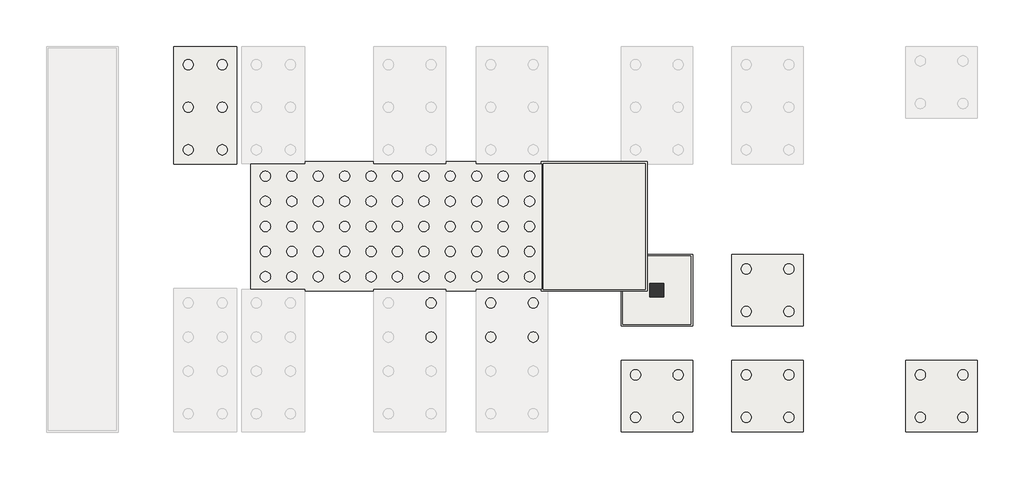
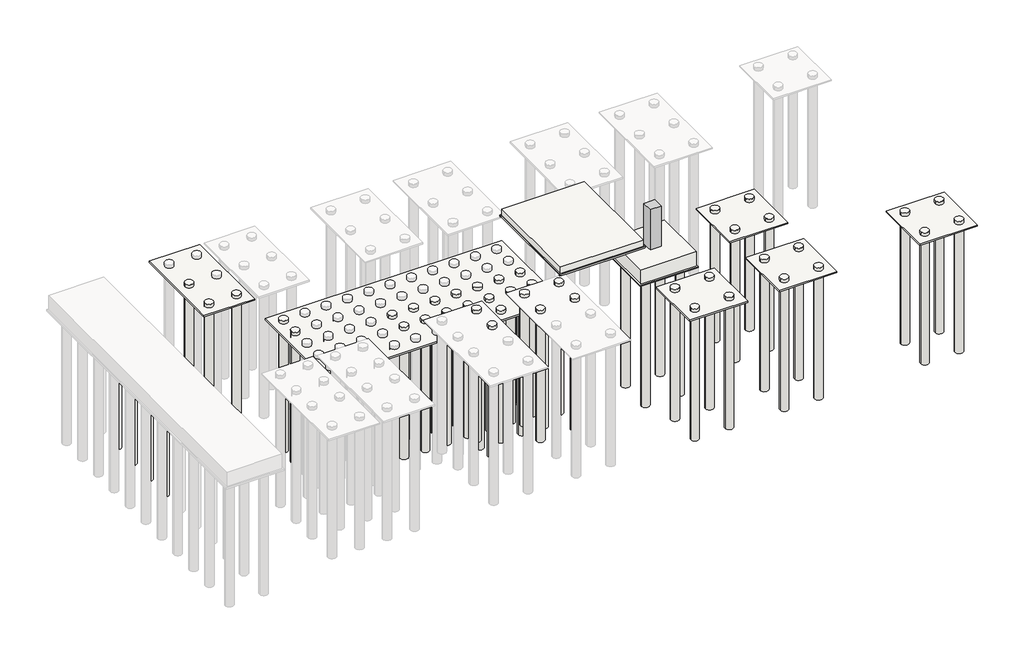
# One storey, part 2 of 3: 63 slabs, 1 column.
"""IFC4 building model written with IfcOpenShell, lengths in millimetres."""

from ifc_helpers import new_model, si_unit, point, frame, frame_2d, origin, place, context, project, spatial, polyline, circle_curve, trimmed, segment, composite_curve, outline, extrude, faceted_brep, element, save

model = new_model("IFC4")

# Units and contexts
model_context = context("Model", 3, world=origin())
ifc_project = project(units=[si_unit("LENGTHUNIT", "METRE", prefix="MILLI")], contexts=[model_context])

# Site, building, storey
site = spatial("IfcSite", under=ifc_project)
building = spatial("IfcBuilding", under=site)
storey = spatial("IfcBuildingStorey", under=building, Name="B.O.F(FDN)", Elevation=-2500.0279945)

# Column
placement = place(None, origin())
element("IfcColumn", 1, ObjectType="RC_Pedestal : H_SC_ACC_PED_W800xL800", at=placement, inside=storey, context=model_context, shape_type="SweptSolid", body=[
    extrude(outline(polyline([(33894.0, 26599.5208589), (33094.0, 26599.5208589), (33094.0, 27399.5208589), (33894.0, 27399.5208589), (33894.0, 26599.5208589)])), frame((0.0, 0.0, -2500.0279945), z_axis=(0.0, 0.0, 1.0), x_axis=(1.0, 0.0, 0.0)), (0.0, 0.0, 1.0), 3100.0),
])

# Slabs
element("IfcSlab", 2, ObjectType="H_SF_ACP_Pit Slab T500", at=placement, inside=storey, context=model_context, shape_type="Brep", body=[
    faceted_brep([(26830.0, 34449.5208589, -2400.0279945), (32830.0, 34449.5208589, -2400.0279945), (32830.0, 27049.5208589, -2400.0279945), (26830.0, 27049.5208589, -2400.0279945), (26830.0, 34449.5208589, -1900.0279945), (26830.0, 34059.5208589, -1900.0279945), (26830.0, 27439.5208589, -1900.0279945), (26830.0, 27049.5208589, -1900.0279945), (32830.0, 27049.5208589, -1900.0279945), (32830.0, 27439.5208589, -1900.0279945), (32830.0, 34059.5208589, -1900.0279945), (32830.0, 34449.5208589, -1900.0279945)], [[[0, 1, 2, 3]], [[4, 5, 6, 7, 8, 9, 10, 11]], [[1, 0, 4, 11]], [[2, 1, 11, 10, 9, 8]], [[3, 2, 8, 7]], [[0, 3, 7, 6, 5, 4]]]),
])
element("IfcSlab", 3, ObjectType="H_SF_ACF_Lean_T100", at=placement, inside=storey, context=model_context, shape_type="SweptSolid", body=[
    extrude(outline(polyline([(48115.0, 22879.5208589), (52315.0, 22879.5208589), (52315.0, 18679.5208589), (48115.0, 18679.5208589), (48115.0, 22879.5208589)])), frame((0.0, 0.0, -2600.0279945), z_axis=(0.0, 0.0, 1.0), x_axis=(1.0, 0.0, 0.0)), (0.0, 0.0, 1.0), 100.0),
])
element("IfcSlab", 4, ObjectType="H_SF_ACF_Lean_T100", at=placement, inside=storey, context=model_context, shape_type="SweptSolid", body=[
    extrude(outline(polyline([(5150.0, 41319.5208589), (8850.0, 41319.5208589), (8850.0, 34399.5208589), (5150.0, 34399.5208589), (5150.0, 41319.5208589)])), frame((0.0, 0.0, -2600.0279945), z_axis=(0.0, 0.0, 1.0), x_axis=(1.0, 0.0, 0.0)), (0.0, 0.0, 1.0), 100.0),
])
element("IfcSlab", 5, ObjectType="H_SF_ACF_Lean_T100", at=placement, inside=storey, context=model_context, shape_type="SweptSolid", body=[
    extrude(outline(polyline([(31400.0, 24899.5208589), (31400.0, 29099.5208589), (35600.0, 29099.5208589), (35600.0, 24899.5208589), (31400.0, 24899.5208589)])), frame((0.0, 0.0, -3700.0279945), z_axis=(0.0, 0.0, 1.0), x_axis=(1.0, 0.0, 0.0)), (0.0, 0.0, 1.0), 100.0),
])
element("IfcSlab", 6, ObjectType="H_SF_ACF_Lean_T100", at=placement, inside=storey, context=model_context, shape_type="Brep", body=[
    faceted_brep([(26730.0, 34549.5208589, -2500.0279945), (27000.0, 34549.5208589, -2500.0279945), (31500.0, 34549.5208589, -2500.0279945), (32930.0, 34549.5208589, -2500.0279945), (32930.0, 34499.5208589, -2500.0279945), (32930.0, 26949.5208589, -2500.0279945), (27000.0, 26949.5208589, -2500.0279945), (26730.0, 26949.5208589, -2500.0279945), (26730.0, 26999.5208589, -2500.0279945), (26730.0, 27049.5208589, -2500.0279945), (26780.0, 27049.5208589, -2500.0279945), (26780.0, 34449.5208589, -2500.0279945), (26730.0, 34449.5208589, -2500.0279945), (26730.0, 34499.5208589, -2500.0279945), (32930.0, 34549.5208589, -2400.0279945), (31500.0, 34549.5208589, -2400.0279945), (27000.0, 34549.5208589, -2400.0279945), (26730.0, 34549.5208589, -2400.0279945), (26730.0, 34499.5208589, -2400.0279945), (26730.0, 34449.5208589, -2400.0279945), (26780.0, 34449.5208589, -2400.0279945), (26780.0, 27049.5208589, -2400.0279945), (26730.0, 27049.5208589, -2400.0279945), (26730.0, 26999.5208589, -2400.0279945), (26730.0, 26949.5208589, -2400.0279945), (27000.0, 26949.5208589, -2400.0279945), (32930.0, 26949.5208589, -2400.0279945), (32930.0, 34499.5208589, -2400.0279945)], [[[0, 1, 2, 3, 4, 5, 6, 7, 8, 9, 10, 11, 12, 13]], [[14, 15, 16, 17, 18, 19, 20, 21, 22, 23, 24, 25, 26, 27]], [[3, 2, 1, 0, 17, 16, 15, 14]], [[5, 4, 3, 14, 27, 26]], [[7, 6, 5, 26, 25, 24]], [[17, 0, 13, 12, 19, 18]], [[7, 24, 23, 22, 9, 8]], [[20, 11, 10, 21]], [[21, 10, 9, 22]], [[11, 20, 19, 12]]]),
])
element("IfcSlab", 7, ObjectType="H_SF_ACF_Lean_T100", at=placement, inside=storey, context=model_context, shape_type="SweptSolid", body=[
    extrude(outline(polyline([(9680.0, 26949.5208589), (9680.0, 34549.5208589), (26880.0, 34549.5208589), (26880.0, 26949.5208589), (9680.0, 26949.5208589)])), frame((0.0, 0.0, -4500.0279945), z_axis=(0.0, 0.0, 1.0), x_axis=(1.0, 0.0, 0.0)), (0.0, 0.0, 1.0), 100.0),
])
element("IfcSlab", 8, ObjectType="H_SF_ACF_Lean_T100", at=placement, inside=storey, context=model_context, shape_type="SweptSolid", body=[
    extrude(outline(polyline([(37900.0, 22879.5208589), (42100.0, 22879.5208589), (42100.0, 18679.5208589), (37900.0, 18679.5208589), (37900.0, 22879.5208589)])), frame((0.0, 0.0, -2600.0279945), z_axis=(0.0, 0.0, 1.0), x_axis=(1.0, 0.0, 0.0)), (0.0, 0.0, 1.0), 100.0),
])
element("IfcSlab", 9, ObjectType="H_SF_ACF_Lean_T100", at=placement, inside=storey, context=model_context, shape_type="SweptSolid", body=[
    extrude(outline(polyline([(31400.0, 22879.5208589), (35600.0, 22879.5208589), (35600.0, 18679.5208589), (31400.0, 18679.5208589), (31400.0, 22879.5208589)])), frame((0.0, 0.0, -2600.0279945), z_axis=(0.0, 0.0, 1.0), x_axis=(1.0, 0.0, 0.0)), (0.0, 0.0, 1.0), 100.0),
])
element("IfcSlab", 10, ObjectType="H_SF_ACF_Lean_T100", at=placement, inside=storey, context=model_context, shape_type="SweptSolid", body=[
    extrude(outline(polyline([(37900.0, 29099.5208589), (42100.0, 29099.5208589), (42100.0, 24899.5208589), (37900.0, 24899.5208589), (37900.0, 29099.5208589)])), frame((0.0, 0.0, -2600.0279945), z_axis=(0.0, 0.0, 1.0), x_axis=(1.0, 0.0, 0.0)), (0.0, 0.0, 1.0), 100.0),
])
element("IfcSlab", 11, ObjectType="Foundation Rectangular(Non-Pile) : H_SF_ACF_W4000xL4000xT1100_Protection", at=placement, inside=storey, context=model_context, shape_type="SweptSolid", body=[
    extrude(outline(polyline([(35500.0, 28999.5208589), (35500.0, 24999.5208589), (31500.0, 24999.5208589), (31500.0, 28999.5208589), (35500.0, 28999.5208589)])), frame((0.0, 0.0, -3600.0279945), z_axis=(0.0, 0.0, 1.0), x_axis=(1.0, 0.0, 0.0)), (0.0, 0.0, 1.0), 1100.0),
])
element("IfcSlab", 12, ObjectType="Pile : H_SF_API_Steel Pile D508x12t_L10m", at=placement, inside=storey, context=model_context, shape_type="SweptSolid", body=[
    extrude(outline(composite_curve([segment(trimmed(circle_curve(frame_2d((1035.0, 38249.5208589)), 300.0), [point((1335.0, 38249.5208589))], [point((735.0, 38249.5208589))], False, "CARTESIAN"), True, "CONTINUOUS"), segment(trimmed(circle_curve(frame_2d((1035.0, 38249.5208589)), 300.0), [point((735.0, 38249.5208589))], [point((1335.0, 38249.5208589))], False, "CARTESIAN"), True, "CONTINUOUS")], self_intersect=False)), frame((0.0, 0.0, -13500.0279945), z_axis=(0.0, 0.0, 1.0), x_axis=(1.0, 0.0, 0.0)), (0.0, 0.0, 1.0), 10150.0),
])
element("IfcSlab", 13, ObjectType="Pile : H_SF_API_Steel Pile D508x12t_L10m", at=placement, inside=storey, context=model_context, shape_type="SweptSolid", body=[
    extrude(outline(composite_curve([segment(trimmed(circle_curve(frame_2d((1035.0, 36249.5208589)), 300.0), [point((1335.0, 36249.5208589))], [point((735.0, 36249.5208589))], False, "CARTESIAN"), True, "CONTINUOUS"), segment(trimmed(circle_curve(frame_2d((1035.0, 36249.5208589)), 300.0), [point((735.0, 36249.5208589))], [point((1335.0, 36249.5208589))], False, "CARTESIAN"), True, "CONTINUOUS")], self_intersect=False)), frame((0.0, 0.0, -13500.0279945), z_axis=(0.0, 0.0, 1.0), x_axis=(1.0, 0.0, 0.0)), (0.0, 0.0, 1.0), 10150.0),
])
element("IfcSlab", 14, ObjectType="Pile : H_SF_API_Steel Pile D508x12t_L10m", at=placement, inside=storey, context=model_context, shape_type="SweptSolid", body=[
    extrude(outline(composite_curve([segment(trimmed(circle_curve(frame_2d((1035.0, 34249.5208589)), 300.0), [point((1335.0, 34249.5208589))], [point((735.0, 34249.5208589))], False, "CARTESIAN"), True, "CONTINUOUS"), segment(trimmed(circle_curve(frame_2d((1035.0, 34249.5208589)), 300.0), [point((735.0, 34249.5208589))], [point((1335.0, 34249.5208589))], False, "CARTESIAN"), True, "CONTINUOUS")], self_intersect=False)), frame((0.0, 0.0, -13500.0279945), z_axis=(0.0, 0.0, 1.0), x_axis=(1.0, 0.0, 0.0)), (0.0, 0.0, 1.0), 10150.0),
])
element("IfcSlab", 15, ObjectType="Pile : H_SF_API_Steel Pile D508x12t_L10m", at=placement, inside=storey, context=model_context, shape_type="SweptSolid", body=[
    extrude(outline(composite_curve([segment(trimmed(circle_curve(frame_2d((1035.0, 32249.5208589)), 300.0), [point((1335.0, 32249.5208589))], [point((735.0, 32249.5208589))], False, "CARTESIAN"), True, "CONTINUOUS"), segment(trimmed(circle_curve(frame_2d((1035.0, 32249.5208589)), 300.0), [point((735.0, 32249.5208589))], [point((1335.0, 32249.5208589))], False, "CARTESIAN"), True, "CONTINUOUS")], self_intersect=False)), frame((0.0, 0.0, -13500.0279945), z_axis=(0.0, 0.0, 1.0), x_axis=(1.0, 0.0, 0.0)), (0.0, 0.0, 1.0), 10150.0),
])
element("IfcSlab", 16, ObjectType="Pile : H_SF_API_Steel Pile D508x12t_L10m", at=placement, inside=storey, context=model_context, shape_type="SweptSolid", body=[
    extrude(outline(composite_curve([segment(trimmed(circle_curve(frame_2d((20250.0, 24249.5208589)), 300.0), [point((20550.0, 24249.5208589))], [point((19950.0, 24249.5208589))], False, "CARTESIAN"), True, "CONTINUOUS"), segment(trimmed(circle_curve(frame_2d((20250.0, 24249.5208589)), 300.0), [point((19950.0, 24249.5208589))], [point((20550.0, 24249.5208589))], False, "CARTESIAN"), True, "CONTINUOUS")], self_intersect=False)), frame((0.0, 0.0, -12400.0279945), z_axis=(0.0, 0.0, 1.0), x_axis=(1.0, 0.0, 0.0)), (0.0, 0.0, 1.0), 10150.0),
])
element("IfcSlab", 17, ObjectType="Pile : H_SF_API_Steel Pile D508x12t_L10m", at=placement, inside=storey, context=model_context, shape_type="SweptSolid", body=[
    extrude(outline(composite_curve([segment(trimmed(circle_curve(frame_2d((20250.0, 26249.5208589)), 300.0), [point((20550.0, 26249.5208589))], [point((19950.0, 26249.5208589))], False, "CARTESIAN"), True, "CONTINUOUS"), segment(trimmed(circle_curve(frame_2d((20250.0, 26249.5208589)), 300.0), [point((19950.0, 26249.5208589))], [point((20550.0, 26249.5208589))], False, "CARTESIAN"), True, "CONTINUOUS")], self_intersect=False)), frame((0.0, 0.0, -12400.0279945), z_axis=(0.0, 0.0, 1.0), x_axis=(1.0, 0.0, 0.0)), (0.0, 0.0, 1.0), 10150.0),
])
element("IfcSlab", 18, ObjectType="Pile : H_SF_API_Steel Pile D508x12t_L10m", at=placement, inside=storey, context=model_context, shape_type="SweptSolid", body=[
    extrude(outline(composite_curve([segment(trimmed(circle_curve(frame_2d((23750.0, 24249.5208589)), 300.0), [point((23450.0, 24249.5208589))], [point((24050.0, 24249.5208589))], False, "CARTESIAN"), True, "CONTINUOUS"), segment(trimmed(circle_curve(frame_2d((23750.0, 24249.5208589)), 300.0), [point((24050.0, 24249.5208589))], [point((23450.0, 24249.5208589))], False, "CARTESIAN"), True, "CONTINUOUS")], self_intersect=False)), frame((0.0, 0.0, -12400.0279945), z_axis=(0.0, 0.0, 1.0), x_axis=(1.0, 0.0, 0.0)), (0.0, 0.0, 1.0), 10150.0),
])
element("IfcSlab", 19, ObjectType="Pile : H_SF_API_Steel Pile D508x12t_L10m", at=placement, inside=storey, context=model_context, shape_type="SweptSolid", body=[
    extrude(outline(composite_curve([segment(trimmed(circle_curve(frame_2d((26250.0, 26249.5208589)), 300.0), [point((26550.0, 26249.5208589))], [point((25950.0, 26249.5208589))], False, "CARTESIAN"), True, "CONTINUOUS"), segment(trimmed(circle_curve(frame_2d((26250.0, 26249.5208589)), 300.0), [point((25950.0, 26249.5208589))], [point((26550.0, 26249.5208589))], False, "CARTESIAN"), True, "CONTINUOUS")], self_intersect=False)), frame((0.0, 0.0, -12400.0279945), z_axis=(0.0, 0.0, 1.0), x_axis=(1.0, 0.0, 0.0)), (0.0, 0.0, 1.0), 10150.0),
])
element("IfcSlab", 20, ObjectType="Pile : H_SF_API_Steel Pile D508x12t_L10m", at=placement, inside=storey, context=model_context, shape_type="SweptSolid", body=[
    extrude(outline(composite_curve([segment(trimmed(circle_curve(frame_2d((23750.0, 26249.5208589)), 300.0), [point((23450.0, 26249.5208589))], [point((24050.0, 26249.5208589))], False, "CARTESIAN"), True, "CONTINUOUS"), segment(trimmed(circle_curve(frame_2d((23750.0, 26249.5208589)), 300.0), [point((24050.0, 26249.5208589))], [point((23450.0, 26249.5208589))], False, "CARTESIAN"), True, "CONTINUOUS")], self_intersect=False)), frame((0.0, 0.0, -12400.0279945), z_axis=(0.0, 0.0, 1.0), x_axis=(1.0, 0.0, 0.0)), (0.0, 0.0, 1.0), 10150.0),
])
element("IfcSlab", 21, ObjectType="Pile : H_SF_API_Steel Pile D508x12t_L10m", at=placement, inside=storey, context=model_context, shape_type="SweptSolid", body=[
    extrude(outline(composite_curve([segment(trimmed(circle_curve(frame_2d((34750.0, 19529.5208589)), 300.0), [point((35050.0, 19529.5208589))], [point((34450.0, 19529.5208589))], False, "CARTESIAN"), True, "CONTINUOUS"), segment(trimmed(circle_curve(frame_2d((34750.0, 19529.5208589)), 300.0), [point((34450.0, 19529.5208589))], [point((35050.0, 19529.5208589))], False, "CARTESIAN"), True, "CONTINUOUS")], self_intersect=False)), frame((0.0, 0.0, -12400.0279945), z_axis=(0.0, 0.0, 1.0), x_axis=(1.0, 0.0, 0.0)), (0.0, 0.0, 1.0), 10150.0),
])
element("IfcSlab", 22, ObjectType="Pile : H_SF_API_Steel Pile D508x12t_L10m", at=placement, inside=storey, context=model_context, shape_type="SweptSolid", body=[
    extrude(outline(composite_curve([segment(trimmed(circle_curve(frame_2d((32250.0, 19529.5208589)), 300.0), [point((31950.0, 19529.5208589))], [point((32550.0, 19529.5208589))], False, "CARTESIAN"), True, "CONTINUOUS"), segment(trimmed(circle_curve(frame_2d((32250.0, 19529.5208589)), 300.0), [point((32550.0, 19529.5208589))], [point((31950.0, 19529.5208589))], False, "CARTESIAN"), True, "CONTINUOUS")], self_intersect=False)), frame((0.0, 0.0, -12400.0279945), z_axis=(0.0, 0.0, 1.0), x_axis=(1.0, 0.0, 0.0)), (0.0, 0.0, 1.0), 10150.0),
])
element("IfcSlab", 23, ObjectType="Pile : H_SF_API_Steel Pile D508x12t_L10m", at=placement, inside=storey, context=model_context, shape_type="SweptSolid", body=[
    extrude(outline(composite_curve([segment(trimmed(circle_curve(frame_2d((34750.0, 22029.5208589)), 300.0), [point((35050.0, 22029.5208589))], [point((34450.0, 22029.5208589))], False, "CARTESIAN"), True, "CONTINUOUS"), segment(trimmed(circle_curve(frame_2d((34750.0, 22029.5208589)), 300.0), [point((34450.0, 22029.5208589))], [point((35050.0, 22029.5208589))], False, "CARTESIAN"), True, "CONTINUOUS")], self_intersect=False)), frame((0.0, 0.0, -12400.0279945), z_axis=(0.0, 0.0, 1.0), x_axis=(1.0, 0.0, 0.0)), (0.0, 0.0, 1.0), 10150.0),
])
element("IfcSlab", 24, ObjectType="Pile : H_SF_API_Steel Pile D508x12t_L10m", at=placement, inside=storey, context=model_context, shape_type="SweptSolid", body=[
    extrude(outline(composite_curve([segment(trimmed(circle_curve(frame_2d((32250.0, 22029.5208589)), 300.0), [point((31950.0, 22029.5208589))], [point((32550.0, 22029.5208589))], False, "CARTESIAN"), True, "CONTINUOUS"), segment(trimmed(circle_curve(frame_2d((32250.0, 22029.5208589)), 300.0), [point((32550.0, 22029.5208589))], [point((31950.0, 22029.5208589))], False, "CARTESIAN"), True, "CONTINUOUS")], self_intersect=False)), frame((0.0, 0.0, -12400.0279945), z_axis=(0.0, 0.0, 1.0), x_axis=(1.0, 0.0, 0.0)), (0.0, 0.0, 1.0), 10150.0),
])
element("IfcSlab", 25, ObjectType="Pile : H_SF_API_Steel Pile D508x12t_L10m", at=placement, inside=storey, context=model_context, shape_type="SweptSolid", body=[
    extrude(outline(composite_curve([segment(trimmed(circle_curve(frame_2d((34750.0, 25749.5208589)), 300.0), [point((35050.0, 25749.5208589))], [point((34450.0, 25749.5208589))], False, "CARTESIAN"), True, "CONTINUOUS"), segment(trimmed(circle_curve(frame_2d((34750.0, 25749.5208589)), 300.0), [point((34450.0, 25749.5208589))], [point((35050.0, 25749.5208589))], False, "CARTESIAN"), True, "CONTINUOUS")], self_intersect=False)), frame((0.0, 0.0, -13600.0279945), z_axis=(0.0, 0.0, 1.0), x_axis=(1.0, 0.0, 0.0)), (0.0, 0.0, 1.0), 10150.0),
])
element("IfcSlab", 26, ObjectType="Pile : H_SF_API_Steel Pile D508x12t_L10m", at=placement, inside=storey, context=model_context, shape_type="SweptSolid", body=[
    extrude(outline(composite_curve([segment(trimmed(circle_curve(frame_2d((32250.0, 25749.5208589)), 300.0), [point((31950.0, 25749.5208589))], [point((32550.0, 25749.5208589))], False, "CARTESIAN"), True, "CONTINUOUS"), segment(trimmed(circle_curve(frame_2d((32250.0, 25749.5208589)), 300.0), [point((32550.0, 25749.5208589))], [point((31950.0, 25749.5208589))], False, "CARTESIAN"), True, "CONTINUOUS")], self_intersect=False)), frame((0.0, 0.0, -13600.0279945), z_axis=(0.0, 0.0, 1.0), x_axis=(1.0, 0.0, 0.0)), (0.0, 0.0, 1.0), 10150.0),
])
element("IfcSlab", 27, ObjectType="Pile : H_SF_API_Steel Pile D508x12t_L10m", at=placement, inside=storey, context=model_context, shape_type="SweptSolid", body=[
    extrude(outline(composite_curve([segment(trimmed(circle_curve(frame_2d((34750.0, 28249.5208589)), 300.0), [point((35050.0, 28249.5208589))], [point((34450.0, 28249.5208589))], False, "CARTESIAN"), True, "CONTINUOUS"), segment(trimmed(circle_curve(frame_2d((34750.0, 28249.5208589)), 300.0), [point((34450.0, 28249.5208589))], [point((35050.0, 28249.5208589))], False, "CARTESIAN"), True, "CONTINUOUS")], self_intersect=False)), frame((0.0, 0.0, -13600.0279945), z_axis=(0.0, 0.0, 1.0), x_axis=(1.0, 0.0, 0.0)), (0.0, 0.0, 1.0), 10150.0),
])
element("IfcSlab", 28, ObjectType="Pile : H_SF_API_Steel Pile D508x12t_L10m", at=placement, inside=storey, context=model_context, shape_type="SweptSolid", body=[
    extrude(outline(composite_curve([segment(trimmed(circle_curve(frame_2d((32250.0, 28249.5208589)), 300.0), [point((31950.0, 28249.5208589))], [point((32550.0, 28249.5208589))], False, "CARTESIAN"), True, "CONTINUOUS"), segment(trimmed(circle_curve(frame_2d((32250.0, 28249.5208589)), 300.0), [point((32550.0, 28249.5208589))], [point((31950.0, 28249.5208589))], False, "CARTESIAN"), True, "CONTINUOUS")], self_intersect=False)), frame((0.0, 0.0, -13600.0279945), z_axis=(0.0, 0.0, 1.0), x_axis=(1.0, 0.0, 0.0)), (0.0, 0.0, 1.0), 10150.0),
])
element("IfcSlab", 29, ObjectType="Pile : H_SF_API_Steel Pile D508x12t_L10m", at=placement, inside=storey, context=model_context, shape_type="SweptSolid", body=[
    extrude(outline(composite_curve([segment(trimmed(circle_curve(frame_2d((41250.0, 25749.5208589)), 300.0), [point((41550.0, 25749.5208589))], [point((40950.0, 25749.5208589))], False, "CARTESIAN"), True, "CONTINUOUS"), segment(trimmed(circle_curve(frame_2d((41250.0, 25749.5208589)), 300.0), [point((40950.0, 25749.5208589))], [point((41550.0, 25749.5208589))], False, "CARTESIAN"), True, "CONTINUOUS")], self_intersect=False)), frame((0.0, 0.0, -12400.0279945), z_axis=(0.0, 0.0, 1.0), x_axis=(1.0, 0.0, 0.0)), (0.0, 0.0, 1.0), 10150.0),
])
element("IfcSlab", 30, ObjectType="Pile : H_SF_API_Steel Pile D508x12t_L10m", at=placement, inside=storey, context=model_context, shape_type="SweptSolid", body=[
    extrude(outline(composite_curve([segment(trimmed(circle_curve(frame_2d((38750.0, 25749.5208589)), 300.0), [point((38450.0, 25749.5208589))], [point((39050.0, 25749.5208589))], False, "CARTESIAN"), True, "CONTINUOUS"), segment(trimmed(circle_curve(frame_2d((38750.0, 25749.5208589)), 300.0), [point((39050.0, 25749.5208589))], [point((38450.0, 25749.5208589))], False, "CARTESIAN"), True, "CONTINUOUS")], self_intersect=False)), frame((0.0, 0.0, -12400.0279945), z_axis=(0.0, 0.0, 1.0), x_axis=(1.0, 0.0, 0.0)), (0.0, 0.0, 1.0), 10150.0),
])
element("IfcSlab", 31, ObjectType="Pile : H_SF_API_Steel Pile D508x12t_L10m", at=placement, inside=storey, context=model_context, shape_type="SweptSolid", body=[
    extrude(outline(composite_curve([segment(trimmed(circle_curve(frame_2d((41250.0, 28249.5208589)), 300.0), [point((41550.0, 28249.5208589))], [point((40950.0, 28249.5208589))], False, "CARTESIAN"), True, "CONTINUOUS"), segment(trimmed(circle_curve(frame_2d((41250.0, 28249.5208589)), 300.0), [point((40950.0, 28249.5208589))], [point((41550.0, 28249.5208589))], False, "CARTESIAN"), True, "CONTINUOUS")], self_intersect=False)), frame((0.0, 0.0, -12400.0279945), z_axis=(0.0, 0.0, 1.0), x_axis=(1.0, 0.0, 0.0)), (0.0, 0.0, 1.0), 10150.0),
])
element("IfcSlab", 32, ObjectType="Pile : H_SF_API_Steel Pile D508x12t_L10m", at=placement, inside=storey, context=model_context, shape_type="SweptSolid", body=[
    extrude(outline(composite_curve([segment(trimmed(circle_curve(frame_2d((38750.0, 28249.5208589)), 300.0), [point((38450.0, 28249.5208589))], [point((39050.0, 28249.5208589))], False, "CARTESIAN"), True, "CONTINUOUS"), segment(trimmed(circle_curve(frame_2d((38750.0, 28249.5208589)), 300.0), [point((39050.0, 28249.5208589))], [point((38450.0, 28249.5208589))], False, "CARTESIAN"), True, "CONTINUOUS")], self_intersect=False)), frame((0.0, 0.0, -12400.0279945), z_axis=(0.0, 0.0, 1.0), x_axis=(1.0, 0.0, 0.0)), (0.0, 0.0, 1.0), 10150.0),
])
element("IfcSlab", 33, ObjectType="Pile : H_SF_API_Steel Pile D508x12t_L10m", at=placement, inside=storey, context=model_context, shape_type="SweptSolid", body=[
    extrude(outline(composite_curve([segment(trimmed(circle_curve(frame_2d((41250.0, 19529.5208589)), 300.0), [point((41550.0, 19529.5208589))], [point((40950.0, 19529.5208589))], False, "CARTESIAN"), True, "CONTINUOUS"), segment(trimmed(circle_curve(frame_2d((41250.0, 19529.5208589)), 300.0), [point((40950.0, 19529.5208589))], [point((41550.0, 19529.5208589))], False, "CARTESIAN"), True, "CONTINUOUS")], self_intersect=False)), frame((0.0, 0.0, -12400.0279945), z_axis=(0.0, 0.0, 1.0), x_axis=(1.0, 0.0, 0.0)), (0.0, 0.0, 1.0), 10150.0),
])
element("IfcSlab", 34, ObjectType="Pile : H_SF_API_Steel Pile D508x12t_L10m", at=placement, inside=storey, context=model_context, shape_type="SweptSolid", body=[
    extrude(outline(composite_curve([segment(trimmed(circle_curve(frame_2d((38750.0, 19529.5208589)), 300.0), [point((38450.0, 19529.5208589))], [point((39050.0, 19529.5208589))], False, "CARTESIAN"), True, "CONTINUOUS"), segment(trimmed(circle_curve(frame_2d((38750.0, 19529.5208589)), 300.0), [point((39050.0, 19529.5208589))], [point((38450.0, 19529.5208589))], False, "CARTESIAN"), True, "CONTINUOUS")], self_intersect=False)), frame((0.0, 0.0, -12400.0279945), z_axis=(0.0, 0.0, 1.0), x_axis=(1.0, 0.0, 0.0)), (0.0, 0.0, 1.0), 10150.0),
])
element("IfcSlab", 35, ObjectType="Pile : H_SF_API_Steel Pile D508x12t_L10m", at=placement, inside=storey, context=model_context, shape_type="SweptSolid", body=[
    extrude(outline(composite_curve([segment(trimmed(circle_curve(frame_2d((41250.0, 22029.5208589)), 300.0), [point((41550.0, 22029.5208589))], [point((40950.0, 22029.5208589))], False, "CARTESIAN"), True, "CONTINUOUS"), segment(trimmed(circle_curve(frame_2d((41250.0, 22029.5208589)), 300.0), [point((40950.0, 22029.5208589))], [point((41550.0, 22029.5208589))], False, "CARTESIAN"), True, "CONTINUOUS")], self_intersect=False)), frame((0.0, 0.0, -12400.0279945), z_axis=(0.0, 0.0, 1.0), x_axis=(1.0, 0.0, 0.0)), (0.0, 0.0, 1.0), 10150.0),
])
element("IfcSlab", 36, ObjectType="Pile : H_SF_API_Steel Pile D508x12t_L10m", at=placement, inside=storey, context=model_context, shape_type="SweptSolid", body=[
    extrude(outline(composite_curve([segment(trimmed(circle_curve(frame_2d((38750.0, 22029.5208589)), 300.0), [point((38450.0, 22029.5208589))], [point((39050.0, 22029.5208589))], False, "CARTESIAN"), True, "CONTINUOUS"), segment(trimmed(circle_curve(frame_2d((38750.0, 22029.5208589)), 300.0), [point((39050.0, 22029.5208589))], [point((38450.0, 22029.5208589))], False, "CARTESIAN"), True, "CONTINUOUS")], self_intersect=False)), frame((0.0, 0.0, -12400.0279945), z_axis=(0.0, 0.0, 1.0), x_axis=(1.0, 0.0, 0.0)), (0.0, 0.0, 1.0), 10150.0),
])
element("IfcSlab", 37, ObjectType="Pile : H_SF_API_Steel Pile D508x12t_L10m", at=placement, inside=storey, context=model_context, shape_type="SweptSolid", body=[
    extrude(outline(composite_curve([segment(trimmed(circle_curve(frame_2d((51465.0, 19529.5208589)), 300.0), [point((51765.0, 19529.5208589))], [point((51165.0, 19529.5208589))], False, "CARTESIAN"), True, "CONTINUOUS"), segment(trimmed(circle_curve(frame_2d((51465.0, 19529.5208589)), 300.0), [point((51165.0, 19529.5208589))], [point((51765.0, 19529.5208589))], False, "CARTESIAN"), True, "CONTINUOUS")], self_intersect=False)), frame((0.0, 0.0, -12400.0279945), z_axis=(0.0, 0.0, 1.0), x_axis=(1.0, 0.0, 0.0)), (0.0, 0.0, 1.0), 10150.0),
])
element("IfcSlab", 38, ObjectType="Pile : H_SF_API_Steel Pile D508x12t_L10m", at=placement, inside=storey, context=model_context, shape_type="SweptSolid", body=[
    extrude(outline(composite_curve([segment(trimmed(circle_curve(frame_2d((48965.0, 19529.5208589)), 300.0), [point((48665.0, 19529.5208589))], [point((49265.0, 19529.5208589))], False, "CARTESIAN"), True, "CONTINUOUS"), segment(trimmed(circle_curve(frame_2d((48965.0, 19529.5208589)), 300.0), [point((49265.0, 19529.5208589))], [point((48665.0, 19529.5208589))], False, "CARTESIAN"), True, "CONTINUOUS")], self_intersect=False)), frame((0.0, 0.0, -12400.0279945), z_axis=(0.0, 0.0, 1.0), x_axis=(1.0, 0.0, 0.0)), (0.0, 0.0, 1.0), 10150.0),
])
element("IfcSlab", 39, ObjectType="Pile : H_SF_API_Steel Pile D508x12t_L10m", at=placement, inside=storey, context=model_context, shape_type="SweptSolid", body=[
    extrude(outline(composite_curve([segment(trimmed(circle_curve(frame_2d((51465.0, 22029.5208589)), 300.0), [point((51765.0, 22029.5208589))], [point((51165.0, 22029.5208589))], False, "CARTESIAN"), True, "CONTINUOUS"), segment(trimmed(circle_curve(frame_2d((51465.0, 22029.5208589)), 300.0), [point((51165.0, 22029.5208589))], [point((51765.0, 22029.5208589))], False, "CARTESIAN"), True, "CONTINUOUS")], self_intersect=False)), frame((0.0, 0.0, -12400.0279945), z_axis=(0.0, 0.0, 1.0), x_axis=(1.0, 0.0, 0.0)), (0.0, 0.0, 1.0), 10150.0),
])
element("IfcSlab", 40, ObjectType="Pile : H_SF_API_Steel Pile D508x12t_L10m", at=placement, inside=storey, context=model_context, shape_type="SweptSolid", body=[
    extrude(outline(composite_curve([segment(trimmed(circle_curve(frame_2d((48965.0, 22029.5208589)), 300.0), [point((48665.0, 22029.5208589))], [point((49265.0, 22029.5208589))], False, "CARTESIAN"), True, "CONTINUOUS"), segment(trimmed(circle_curve(frame_2d((48965.0, 22029.5208589)), 300.0), [point((49265.0, 22029.5208589))], [point((48665.0, 22029.5208589))], False, "CARTESIAN"), True, "CONTINUOUS")], self_intersect=False)), frame((0.0, 0.0, -12400.0279945), z_axis=(0.0, 0.0, 1.0), x_axis=(1.0, 0.0, 0.0)), (0.0, 0.0, 1.0), 10150.0),
])
element("IfcSlab", 41, ObjectType="Pile : H_SF_API_Steel Pile D508x12t_L10m", at=placement, inside=storey, context=model_context, shape_type="SweptSolid", body=[
    extrude(outline(composite_curve([segment(trimmed(circle_curve(frame_2d((6000.0, 37749.5208589)), 300.0), [point((5700.0, 37749.5208589))], [point((6300.0, 37749.5208589))], False, "CARTESIAN"), True, "CONTINUOUS"), segment(trimmed(circle_curve(frame_2d((6000.0, 37749.5208589)), 300.0), [point((6300.0, 37749.5208589))], [point((5700.0, 37749.5208589))], False, "CARTESIAN"), True, "CONTINUOUS")], self_intersect=False)), frame((0.0, 0.0, -12400.0279945), z_axis=(0.0, 0.0, 1.0), x_axis=(1.0, 0.0, 0.0)), (0.0, 0.0, 1.0), 10150.0),
])
element("IfcSlab", 42, ObjectType="Pile : H_SF_API_Steel Pile D508x12t_L10m", at=placement, inside=storey, context=model_context, shape_type="SweptSolid", body=[
    extrude(outline(composite_curve([segment(trimmed(circle_curve(frame_2d((6000.0, 35249.5208589)), 300.0), [point((5700.0, 35249.5208589))], [point((6300.0, 35249.5208589))], False, "CARTESIAN"), True, "CONTINUOUS"), segment(trimmed(circle_curve(frame_2d((6000.0, 35249.5208589)), 300.0), [point((6300.0, 35249.5208589))], [point((5700.0, 35249.5208589))], False, "CARTESIAN"), True, "CONTINUOUS")], self_intersect=False)), frame((0.0, 0.0, -12400.0279945), z_axis=(0.0, 0.0, 1.0), x_axis=(1.0, 0.0, 0.0)), (0.0, 0.0, 1.0), 10150.0),
])
element("IfcSlab", 43, ObjectType="Pile : H_SF_API_Steel Pile D508x12t_L10m", at=placement, inside=storey, context=model_context, shape_type="SweptSolid", body=[
    extrude(outline(composite_curve([segment(trimmed(circle_curve(frame_2d((8000.0, 35249.5208589)), 300.0), [point((8300.0, 35249.5208589))], [point((7700.0, 35249.5208589))], False, "CARTESIAN"), True, "CONTINUOUS"), segment(trimmed(circle_curve(frame_2d((8000.0, 35249.5208589)), 300.0), [point((7700.0, 35249.5208589))], [point((8300.0, 35249.5208589))], False, "CARTESIAN"), True, "CONTINUOUS")], self_intersect=False)), frame((0.0, 0.0, -12400.0279945), z_axis=(0.0, 0.0, 1.0), x_axis=(1.0, 0.0, 0.0)), (0.0, 0.0, 1.0), 10150.0),
])
element("IfcSlab", 44, ObjectType="Pile : H_SF_API_Steel Pile D508x12t_L10m", at=placement, inside=storey, context=model_context, shape_type="SweptSolid", body=[
    extrude(outline(composite_curve([segment(trimmed(circle_curve(frame_2d((10530.0, 33699.5208589)), 300.0), [point((10230.0, 33699.5208589))], [point((10830.0, 33699.5208589))], False, "CARTESIAN"), True, "CONTINUOUS"), segment(trimmed(circle_curve(frame_2d((10530.0, 33699.5208589)), 300.0), [point((10830.0, 33699.5208589))], [point((10230.0, 33699.5208589))], False, "CARTESIAN"), True, "CONTINUOUS")], self_intersect=False)), frame((0.0, 0.0, -14300.0279945), z_axis=(0.0, 0.0, 1.0), x_axis=(1.0, 0.0, 0.0)), (0.0, 0.0, 1.0), 10150.0),
])
element("IfcSlab", 45, ObjectType="Pile : H_SF_API_Steel Pile D508x12t_L10m", at=placement, inside=storey, context=model_context, shape_type="SweptSolid", body=[
    extrude(outline(composite_curve([segment(trimmed(circle_curve(frame_2d((10530.0, 32224.5208589)), 300.0), [point((10230.0, 32224.5208589))], [point((10830.0, 32224.5208589))], False, "CARTESIAN"), True, "CONTINUOUS"), segment(trimmed(circle_curve(frame_2d((10530.0, 32224.5208589)), 300.0), [point((10830.0, 32224.5208589))], [point((10230.0, 32224.5208589))], False, "CARTESIAN"), True, "CONTINUOUS")], self_intersect=False)), frame((0.0, 0.0, -14300.0279945), z_axis=(0.0, 0.0, 1.0), x_axis=(1.0, 0.0, 0.0)), (0.0, 0.0, 1.0), 10150.0),
])
element("IfcSlab", 46, ObjectType="Pile : H_SF_API_Steel Pile D508x12t_L10m", at=placement, inside=storey, context=model_context, shape_type="SweptSolid", body=[
    extrude(outline(composite_curve([segment(trimmed(circle_curve(frame_2d((26030.0, 27799.5208589)), 300.0), [point((26330.0, 27799.5208589))], [point((25730.0, 27799.5208589))], False, "CARTESIAN"), True, "CONTINUOUS"), segment(trimmed(circle_curve(frame_2d((26030.0, 27799.5208589)), 300.0), [point((25730.0, 27799.5208589))], [point((26330.0, 27799.5208589))], False, "CARTESIAN"), True, "CONTINUOUS")], self_intersect=False)), frame((0.0, 0.0, -14300.0279945), z_axis=(0.0, 0.0, 1.0), x_axis=(1.0, 0.0, 0.0)), (0.0, 0.0, 1.0), 10150.0),
])
element("IfcSlab", 47, ObjectType="Pile : H_SF_API_Steel Pile D508x12t_L10m", at=placement, inside=storey, context=model_context, shape_type="SweptSolid", body=[
    extrude(outline(composite_curve([segment(trimmed(circle_curve(frame_2d((26030.0, 29274.5208589)), 300.0), [point((26330.0, 29274.5208589))], [point((25730.0, 29274.5208589))], False, "CARTESIAN"), True, "CONTINUOUS"), segment(trimmed(circle_curve(frame_2d((26030.0, 29274.5208589)), 300.0), [point((25730.0, 29274.5208589))], [point((26330.0, 29274.5208589))], False, "CARTESIAN"), True, "CONTINUOUS")], self_intersect=False)), frame((0.0, 0.0, -14300.0279945), z_axis=(0.0, 0.0, 1.0), x_axis=(1.0, 0.0, 0.0)), (0.0, 0.0, 1.0), 10150.0),
])
element("IfcSlab", 48, ObjectType="Pile : H_SF_API_Steel Pile D508x12t_L10m", at=placement, inside=storey, context=model_context, shape_type="SweptSolid", body=[
    extrude(outline(composite_curve([segment(trimmed(circle_curve(frame_2d((26030.0, 30749.5208589)), 300.0), [point((26330.0, 30749.5208589))], [point((25730.0, 30749.5208589))], False, "CARTESIAN"), True, "CONTINUOUS"), segment(trimmed(circle_curve(frame_2d((26030.0, 30749.5208589)), 300.0), [point((25730.0, 30749.5208589))], [point((26330.0, 30749.5208589))], False, "CARTESIAN"), True, "CONTINUOUS")], self_intersect=False)), frame((0.0, 0.0, -14300.0279945), z_axis=(0.0, 0.0, 1.0), x_axis=(1.0, 0.0, 0.0)), (0.0, 0.0, 1.0), 10150.0),
])
element("IfcSlab", 49, ObjectType="Pile : H_SF_API_Steel Pile D508x12t_L10m", at=placement, inside=storey, context=model_context, shape_type="SweptSolid", body=[
    extrude(outline(composite_curve([segment(trimmed(circle_curve(frame_2d((24480.0, 27799.5208589)), 300.0), [point((24780.0, 27799.5208589))], [point((24180.0, 27799.5208589))], False, "CARTESIAN"), True, "CONTINUOUS"), segment(trimmed(circle_curve(frame_2d((24480.0, 27799.5208589)), 300.0), [point((24180.0, 27799.5208589))], [point((24780.0, 27799.5208589))], False, "CARTESIAN"), True, "CONTINUOUS")], self_intersect=False)), frame((0.0, 0.0, -14300.0279945), z_axis=(0.0, 0.0, 1.0), x_axis=(1.0, 0.0, 0.0)), (0.0, 0.0, 1.0), 10150.0),
])
element("IfcSlab", 50, ObjectType="Pile : H_SF_API_Steel Pile D508x12t_L10m", at=placement, inside=storey, context=model_context, shape_type="SweptSolid", body=[
    extrude(outline(composite_curve([segment(trimmed(circle_curve(frame_2d((24480.0, 29274.5208589)), 300.0), [point((24780.0, 29274.5208589))], [point((24180.0, 29274.5208589))], False, "CARTESIAN"), True, "CONTINUOUS"), segment(trimmed(circle_curve(frame_2d((24480.0, 29274.5208589)), 300.0), [point((24180.0, 29274.5208589))], [point((24780.0, 29274.5208589))], False, "CARTESIAN"), True, "CONTINUOUS")], self_intersect=False)), frame((0.0, 0.0, -14300.0279945), z_axis=(0.0, 0.0, 1.0), x_axis=(1.0, 0.0, 0.0)), (0.0, 0.0, 1.0), 10150.0),
])
element("IfcSlab", 51, ObjectType="Pile : H_SF_API_Steel Pile D508x12t_L10m", at=placement, inside=storey, context=model_context, shape_type="SweptSolid", body=[
    extrude(outline(composite_curve([segment(trimmed(circle_curve(frame_2d((24480.0, 30749.5208589)), 300.0), [point((24780.0, 30749.5208589))], [point((24180.0, 30749.5208589))], False, "CARTESIAN"), True, "CONTINUOUS"), segment(trimmed(circle_curve(frame_2d((24480.0, 30749.5208589)), 300.0), [point((24180.0, 30749.5208589))], [point((24780.0, 30749.5208589))], False, "CARTESIAN"), True, "CONTINUOUS")], self_intersect=False)), frame((0.0, 0.0, -14300.0279945), z_axis=(0.0, 0.0, 1.0), x_axis=(1.0, 0.0, 0.0)), (0.0, 0.0, 1.0), 10150.0),
])
element("IfcSlab", 52, ObjectType="Pile : H_SF_API_Steel Pile D508x12t_L10m", at=placement, inside=storey, context=model_context, shape_type="SweptSolid", body=[
    extrude(outline(composite_curve([segment(trimmed(circle_curve(frame_2d((22930.0, 27799.5208589)), 300.0), [point((23230.0, 27799.5208589))], [point((22630.0, 27799.5208589))], False, "CARTESIAN"), True, "CONTINUOUS"), segment(trimmed(circle_curve(frame_2d((22930.0, 27799.5208589)), 300.0), [point((22630.0, 27799.5208589))], [point((23230.0, 27799.5208589))], False, "CARTESIAN"), True, "CONTINUOUS")], self_intersect=False)), frame((0.0, 0.0, -14300.0279945), z_axis=(0.0, 0.0, 1.0), x_axis=(1.0, 0.0, 0.0)), (0.0, 0.0, 1.0), 10150.0),
])
element("IfcSlab", 53, ObjectType="Pile : H_SF_API_Steel Pile D508x12t_L10m", at=placement, inside=storey, context=model_context, shape_type="SweptSolid", body=[
    extrude(outline(composite_curve([segment(trimmed(circle_curve(frame_2d((22930.0, 29274.5208589)), 300.0), [point((23230.0, 29274.5208589))], [point((22630.0, 29274.5208589))], False, "CARTESIAN"), True, "CONTINUOUS"), segment(trimmed(circle_curve(frame_2d((22930.0, 29274.5208589)), 300.0), [point((22630.0, 29274.5208589))], [point((23230.0, 29274.5208589))], False, "CARTESIAN"), True, "CONTINUOUS")], self_intersect=False)), frame((0.0, 0.0, -14300.0279945), z_axis=(0.0, 0.0, 1.0), x_axis=(1.0, 0.0, 0.0)), (0.0, 0.0, 1.0), 10150.0),
])
element("IfcSlab", 54, ObjectType="Pile : H_SF_API_Steel Pile D508x12t_L10m", at=placement, inside=storey, context=model_context, shape_type="SweptSolid", body=[
    extrude(outline(composite_curve([segment(trimmed(circle_curve(frame_2d((22930.0, 30749.5208589)), 300.0), [point((23230.0, 30749.5208589))], [point((22630.0, 30749.5208589))], False, "CARTESIAN"), True, "CONTINUOUS"), segment(trimmed(circle_curve(frame_2d((22930.0, 30749.5208589)), 300.0), [point((22630.0, 30749.5208589))], [point((23230.0, 30749.5208589))], False, "CARTESIAN"), True, "CONTINUOUS")], self_intersect=False)), frame((0.0, 0.0, -14300.0279945), z_axis=(0.0, 0.0, 1.0), x_axis=(1.0, 0.0, 0.0)), (0.0, 0.0, 1.0), 10150.0),
])
element("IfcSlab", 55, ObjectType="Pile : H_SF_API_Steel Pile D508x12t_L10m", at=placement, inside=storey, context=model_context, shape_type="SweptSolid", body=[
    extrude(outline(composite_curve([segment(trimmed(circle_curve(frame_2d((21380.0, 27799.5208589)), 300.0), [point((21680.0, 27799.5208589))], [point((21080.0, 27799.5208589))], False, "CARTESIAN"), True, "CONTINUOUS"), segment(trimmed(circle_curve(frame_2d((21380.0, 27799.5208589)), 300.0), [point((21080.0, 27799.5208589))], [point((21680.0, 27799.5208589))], False, "CARTESIAN"), True, "CONTINUOUS")], self_intersect=False)), frame((0.0, 0.0, -14300.0279945), z_axis=(0.0, 0.0, 1.0), x_axis=(1.0, 0.0, 0.0)), (0.0, 0.0, 1.0), 10150.0),
])
element("IfcSlab", 56, ObjectType="Pile : H_SF_API_Steel Pile D508x12t_L10m", at=placement, inside=storey, context=model_context, shape_type="SweptSolid", body=[
    extrude(outline(composite_curve([segment(trimmed(circle_curve(frame_2d((21380.0, 29274.5208589)), 300.0), [point((21680.0, 29274.5208589))], [point((21080.0, 29274.5208589))], False, "CARTESIAN"), True, "CONTINUOUS"), segment(trimmed(circle_curve(frame_2d((21380.0, 29274.5208589)), 300.0), [point((21080.0, 29274.5208589))], [point((21680.0, 29274.5208589))], False, "CARTESIAN"), True, "CONTINUOUS")], self_intersect=False)), frame((0.0, 0.0, -14300.0279945), z_axis=(0.0, 0.0, 1.0), x_axis=(1.0, 0.0, 0.0)), (0.0, 0.0, 1.0), 10150.0),
])
element("IfcSlab", 57, ObjectType="Pile : H_SF_API_Steel Pile D508x12t_L10m", at=placement, inside=storey, context=model_context, shape_type="SweptSolid", body=[
    extrude(outline(composite_curve([segment(trimmed(circle_curve(frame_2d((21380.0, 30749.5208589)), 300.0), [point((21680.0, 30749.5208589))], [point((21080.0, 30749.5208589))], False, "CARTESIAN"), True, "CONTINUOUS"), segment(trimmed(circle_curve(frame_2d((21380.0, 30749.5208589)), 300.0), [point((21080.0, 30749.5208589))], [point((21680.0, 30749.5208589))], False, "CARTESIAN"), True, "CONTINUOUS")], self_intersect=False)), frame((0.0, 0.0, -14300.0279945), z_axis=(0.0, 0.0, 1.0), x_axis=(1.0, 0.0, 0.0)), (0.0, 0.0, 1.0), 10150.0),
])
element("IfcSlab", 58, ObjectType="Pile : H_SF_API_Steel Pile D508x12t_L10m", at=placement, inside=storey, context=model_context, shape_type="SweptSolid", body=[
    extrude(outline(composite_curve([segment(trimmed(circle_curve(frame_2d((19830.0, 29274.5208589)), 300.0), [point((20130.0, 29274.5208589))], [point((19530.0, 29274.5208589))], False, "CARTESIAN"), True, "CONTINUOUS"), segment(trimmed(circle_curve(frame_2d((19830.0, 29274.5208589)), 300.0), [point((19530.0, 29274.5208589))], [point((20130.0, 29274.5208589))], False, "CARTESIAN"), True, "CONTINUOUS")], self_intersect=False)), frame((0.0, 0.0, -14300.0279945), z_axis=(0.0, 0.0, 1.0), x_axis=(1.0, 0.0, 0.0)), (0.0, 0.0, 1.0), 10150.0),
])
element("IfcSlab", 59, ObjectType="Pile : H_SF_API_Steel Pile D508x12t_L10m", at=placement, inside=storey, context=model_context, shape_type="SweptSolid", body=[
    extrude(outline(composite_curve([segment(trimmed(circle_curve(frame_2d((19830.0, 30749.5208589)), 300.0), [point((20130.0, 30749.5208589))], [point((19530.0, 30749.5208589))], False, "CARTESIAN"), True, "CONTINUOUS"), segment(trimmed(circle_curve(frame_2d((19830.0, 30749.5208589)), 300.0), [point((19530.0, 30749.5208589))], [point((20130.0, 30749.5208589))], False, "CARTESIAN"), True, "CONTINUOUS")], self_intersect=False)), frame((0.0, 0.0, -14300.0279945), z_axis=(0.0, 0.0, 1.0), x_axis=(1.0, 0.0, 0.0)), (0.0, 0.0, 1.0), 10150.0),
])
element("IfcSlab", 60, ObjectType="Pile : H_SF_API_Steel Pile D508x12t_L10m", at=placement, inside=storey, context=model_context, shape_type="SweptSolid", body=[
    extrude(outline(composite_curve([segment(trimmed(circle_curve(frame_2d((18280.0, 29274.5208589)), 300.0), [point((18580.0, 29274.5208589))], [point((17980.0, 29274.5208589))], False, "CARTESIAN"), True, "CONTINUOUS"), segment(trimmed(circle_curve(frame_2d((18280.0, 29274.5208589)), 300.0), [point((17980.0, 29274.5208589))], [point((18580.0, 29274.5208589))], False, "CARTESIAN"), True, "CONTINUOUS")], self_intersect=False)), frame((0.0, 0.0, -14300.0279945), z_axis=(0.0, 0.0, 1.0), x_axis=(1.0, 0.0, 0.0)), (0.0, 0.0, 1.0), 10150.0),
])
element("IfcSlab", 61, ObjectType="Pile : H_SF_API_Steel Pile D508x12t_L10m", at=placement, inside=storey, context=model_context, shape_type="SweptSolid", body=[
    extrude(outline(composite_curve([segment(trimmed(circle_curve(frame_2d((18280.0, 30749.5208589)), 300.0), [point((18580.0, 30749.5208589))], [point((17980.0, 30749.5208589))], False, "CARTESIAN"), True, "CONTINUOUS"), segment(trimmed(circle_curve(frame_2d((18280.0, 30749.5208589)), 300.0), [point((17980.0, 30749.5208589))], [point((18580.0, 30749.5208589))], False, "CARTESIAN"), True, "CONTINUOUS")], self_intersect=False)), frame((0.0, 0.0, -14300.0279945), z_axis=(0.0, 0.0, 1.0), x_axis=(1.0, 0.0, 0.0)), (0.0, 0.0, 1.0), 10150.0),
])
element("IfcSlab", 62, ObjectType="Pile : H_SF_API_Steel Pile D508x12t_L10m", at=placement, inside=storey, context=model_context, shape_type="SweptSolid", body=[
    extrude(outline(composite_curve([segment(trimmed(circle_curve(frame_2d((16730.0, 29274.5208589)), 300.0), [point((17030.0, 29274.5208589))], [point((16430.0, 29274.5208589))], False, "CARTESIAN"), True, "CONTINUOUS"), segment(trimmed(circle_curve(frame_2d((16730.0, 29274.5208589)), 300.0), [point((16430.0, 29274.5208589))], [point((17030.0, 29274.5208589))], False, "CARTESIAN"), True, "CONTINUOUS")], self_intersect=False)), frame((0.0, 0.0, -14300.0279945), z_axis=(0.0, 0.0, 1.0), x_axis=(1.0, 0.0, 0.0)), (0.0, 0.0, 1.0), 10150.0),
])
element("IfcSlab", 63, ObjectType="Pile : H_SF_API_Steel Pile D508x12t_L10m", at=placement, inside=storey, context=model_context, shape_type="SweptSolid", body=[
    extrude(outline(composite_curve([segment(trimmed(circle_curve(frame_2d((16730.0, 30749.5208589)), 300.0), [point((17030.0, 30749.5208589))], [point((16430.0, 30749.5208589))], False, "CARTESIAN"), True, "CONTINUOUS"), segment(trimmed(circle_curve(frame_2d((16730.0, 30749.5208589)), 300.0), [point((16430.0, 30749.5208589))], [point((17030.0, 30749.5208589))], False, "CARTESIAN"), True, "CONTINUOUS")], self_intersect=False)), frame((0.0, 0.0, -14300.0279945), z_axis=(0.0, 0.0, 1.0), x_axis=(1.0, 0.0, 0.0)), (0.0, 0.0, 1.0), 10150.0),
])
element("IfcSlab", 64, ObjectType="Pile : H_SF_API_Steel Pile D508x12t_L10m", at=placement, inside=storey, context=model_context, shape_type="SweptSolid", body=[
    extrude(outline(composite_curve([segment(trimmed(circle_curve(frame_2d((26250.0, 24249.5208589)), 300.0), [point((25950.0, 24249.5208589))], [point((26550.0, 24249.5208589))], False, "CARTESIAN"), True, "CONTINUOUS"), segment(trimmed(circle_curve(frame_2d((26250.0, 24249.5208589)), 300.0), [point((26550.0, 24249.5208589))], [point((25950.0, 24249.5208589))], False, "CARTESIAN"), True, "CONTINUOUS")], self_intersect=False)), frame((0.0, 0.0, -12400.0279945), z_axis=(0.0, 0.0, 1.0), x_axis=(1.0, 0.0, 0.0)), (0.0, 0.0, 1.0), 10150.0),
])

save(model, "model.ifc")

# Revit data of these elements
# Type "RC_Pedestal : H_SC_ACC_PED_W800xL800"
#   H_WM Code_1 = "A03AD032-00012 | Concrete Work | Substructure Work | Structural Concrete | Cement Type-5 | 20MPa < F'c (Cylinder Strength) ≤ 25MPa"
#   H_WM Code_2 = "A03AD037-00002 | Concrete Work | Substructure Work | Rebar Work | Deformed Bar (Non-Coat.) | 400MPa<Fy≤470MPa"
#   H_WM Code_3 = "A03AD035-00001 | Concrete Work | Substructure Work | Form Work (3 times in use) | Flat Form | Dressed Lumber, Plywood or Steel Form(Wood Planks are not Allowed) incl. Chamfer"
#   H_WM Code_4 = "A03AH056-00001 | Concrete Work | Concrete Protective Coating (U/G) | Bitumen/Bituminous/Asphalt Coating"
#   H_Q'ty Cal Type Tag = "SC-Q1"
#   Description = "AG RC 기둥"
#   Width = 0.8000 m
#   Length = 0.8000 m
#   hec_material3 [instance default] = none
#   hec_material2 [instance default] = A04AM078-00002_Int Wall Painting_Water Emulsion Paint
#   hec_material1 [instance default] = A03AD036-00001_Form Work (1 time in use)
#   Structural Material [instance default] = A03AD032-00007_Structural Concrete_25MPa-30MPa
# Type "H_SF_ACP_Pit Slab T500"
#   Type Comments = ""
#   Type Mark = ""
#   H_WM Code_1 = "A03AD032-00012 | Concrete Work | Substructure Work | Structural Concrete | Cement Type-5 | 20MPa < F'c (Cylinder Strength) ≤ 25MPa"
#   H_WM Code_2 = "A03AD037-00002 | Concrete Work | Substructure Work | Rebar Work | Deformed Bar (Non-Coat.) | 400MPa<Fy≤470MPa"
#   H_WM Code_3 = "A03AD035-00001 | Concrete Work | Substructure Work | Form Work (3 times in use) | Flat Form | Dressed Lumber, Plywood or Steel Form(Wood Planks are not Allowed) incl. Chamfer"
#   H_Q'ty Cal Type Tag = "SF-Q1"
#   Layers, outside or top first: 0.5000 m "A03AG032-00004_Structural Concrete_Type-1_30Mpa" (function 1)
# Type "H_SF_ACF_Lean_T100"
#   Type Comments = "구조_콘크리트"
#   H_WM Code_1 = "A03AD034-00004 | Concrete Work | Substructure Work | Lean Concrete (including Form work) | Cement Type-1 | 10MPa < F'c (Cylinder Strength) ≤ 20MPa"
#   H_WM Code_2 = "A01ZZ005-00001 | Earth Work | - | Base Course | THK≤150mm | THK=(  )mm | CBR=(  )%"
#   H_WM Code_3 = "A01ZZ006-00001 | Earth Work | - | Subbase Course | Including Compaction of Sub-Grade | THK≤150mm | THK=(  )mm | CBR=(  )% for Subgrade, (  )% for Subbase | Compaction=(  )% for Subgrade, (  )% for Subbase"
#   H_WM Code_4 = "A01ZZ012-00001 | Earth Work | - | PE Sheet (Vapor Barrier) | THK=(  )mm"
#   H_Q'ty Cal Type Tag = "SF-Q3"
#   Layers, outside or top first: 0.1000 m "A03AC034-00004_Lean Concrete (including Form work)" (function 1)
# Type "Foundation Rectangular(Non-Pile) : H_SF_ACF_W4000xL4000xT1100_Protection"
#   H_WM Code_1 = "A03AD032-00012 | Concrete Work | Substructure Work | Structural Concrete | Cement Type-5 | 20MPa < F'c (Cylinder Strength) ≤ 25MPa"
#   H_WM Code_2 = "A03AD037-00002 | Concrete Work | Substructure Work | Rebar Work | Deformed Bar (Non-Coat.) | 400MPa<Fy≤470MPa"
#   H_WM Code_3 = "A03AD035-00001 | Concrete Work | Substructure Work | Form Work (3 times in use) | Flat Form | Dressed Lumber, Plywood or Steel Form(Wood Planks are not Allowed) incl. Chamfer"
#   H_WM Code_4 = "A03AH056-00001 | Concrete Work | Concrete Protective Coating (U/G) | Bitumen/Bituminous/Asphalt Coating"
#   H_WM Code_5 = "A03AH059-00001 | Concrete Work | Concrete Protective Coating (U/G) | Sheet Membrane | Adhesive Rubber Sheet or Bitumen Polyethylene Laminated Waterproofing Membrane | THK=(  )mm"
#   H_WM Code_6 = "A03AH060-00001 | Concrete Work | Concrete Protective Coating (U/G) | Memebrane Protection Board | Bitumen Impregnated Fiberboard | THK=(  )mm"
#   H_WM Code_7 = "A01ZZ001-00005 | Earth Work | - | Excavation | Soil, Mech. | 2.0M < D ≤ 4.0M"
#   H_WM Code_8 = "A01ZZ003-00001 | Earth Work | - | Backfill | Re-use, Soil | Compaction=(  )%"
#   H_WM Code_9 = "A01ZZ004-00001 | Earth Work | - | Disposal | Soil | Disposal Distance=Appx. (  )km from Site"
#   H_Q'ty Cal Type Tag = "SF-Q4"
#   Top bar = "D25@300"
#   Description = "UG Shallow Foundation"
#   Bottom bar = "D20@300"
#   Width = 4.0000 m
#   Length = 4.0000 m
#   Foundation Thickness = 1.1000 m
#   Structural Material [instance default] = A03AD032-00010_Structural Concrete_UG_20-24MPa
#   Assembly Code = ""
# Type "Pile : H_SF_API_Steel Pile D508x12t_L10m"
#   Type Mark = ""
#   H_WM Code_1 = "A02AA020-00001 | Pile Work | Piling Work | Steel Pipe Pile Work | Direct Driving | Including Pile Connection and Joint Welding Work | D=(  )mm / THK=(  )mm | Pile Length per Hole=(  )M"
#   H_WM Code_2 = "A02AB020-00001 | Pile Work | Pile Head Treatment | Steel Pipe Pile Work | D=(  )mm / THK=(  )mm"
#   H_Q'ty Cal Type Tag = "SF-Q5"
#   Assembly Code = "A1020130"
#   반지름 = 0.3000 m
#   최소 내포 = 0.1500 m
#   Diameter = 0.6000 m
#   Depth = 10.0000 m
#   VISIBLE [instance default] = yes
#   구조 재료 = 콘크리트
# Element 1 (IfcColumn, "RC_Pedestal : H_SC_ACC_PED_W800xL800")
#   Mark = "PD1"
#   hec_material3 = none
#   hec_material2 = none
#   hec_material1 = none
#   Structural Material = A03AD032-00010_Structural Concrete_UG_20-24MPa
#   Phase Created = New Construction
#   Materials on its faces: "A03AD032-00010_Structural Concrete_UG_20-24MPa"
# Element 2 (IfcSlab, "H_SF_ACP_Pit Slab T500")
#   Comments = ""
#   Mark = "PF1"
#   built-in parameter 1001955 = 3.14159 (stored number, unit not read)
#   Height Offset From Level = 0.6000 m
#   built-in parameter 1001954 = 1
#   Phase Created = New Construction
#   Materials on its faces: "A03AG032-00004_Structural Concrete_Type-1_30Mpa"
# Elements 3, 4, 8, 9, 10 (IfcSlab, "H_SF_ACF_Lean_T100")
#   Comments = ""
#   built-in parameter 1001955 = 3.14159 (stored number, unit not read)
#   Height Offset From Level = 0.0000 m
#   built-in parameter 1001954 = 1
#   Phase Created = New Construction
#   Materials on its faces: "A03AC034-00004_Lean Concrete (including Form work)"
# Element 5 (IfcSlab, "H_SF_ACF_Lean_T100")
#   Comments = ""
#   built-in parameter 1001955 = 3.14159 (stored number, unit not read)
#   Height Offset From Level = -1.1000 m
#   built-in parameter 1001954 = 1
#   Phase Created = New Construction
#   Materials on its faces: "A03AC034-00004_Lean Concrete (including Form work)"
# Element 6 (IfcSlab, "H_SF_ACF_Lean_T100")
#   Comments = ""
#   built-in parameter 1001955 = 3.14159 (stored number, unit not read)
#   Height Offset From Level = 0.1000 m
#   built-in parameter 1001954 = 1
#   Phase Created = New Construction
#   Materials on its faces: "A03AC034-00004_Lean Concrete (including Form work)"
# Element 7 (IfcSlab, "H_SF_ACF_Lean_T100")
#   Comments = ""
#   built-in parameter 1001955 = 3.14159 (stored number, unit not read)
#   Height Offset From Level = -1.9000 m
#   built-in parameter 1001954 = 1
#   Phase Created = New Construction
#   Materials on its faces: "A03AC034-00004_Lean Concrete (including Form work)"
# Element 11 (IfcSlab, "Foundation Rectangular(Non-Pile) : H_SF_ACF_W4000xL4000xT1100_Protection")
#   Comments = ""
#   Mark = "F7"
#   Structural Material = A03AD032-00010_Structural Concrete_UG_20-24MPa
#   Phase Created = New Construction
#   Materials on its faces: "A03AD032-00010_Structural Concrete_UG_20-24MPa"
# Element 12 (IfcSlab, "Pile : H_SF_API_Steel Pile D508x12t_L10m")
#   Mark = "104"
#   Phase Created = New Construction
#   Materials on its faces: "금속 - 스틸 - 345MPa"
# Element 13 (IfcSlab, "Pile : H_SF_API_Steel Pile D508x12t_L10m")
#   Mark = "106"
#   Phase Created = New Construction
#   Materials on its faces: "금속 - 스틸 - 345MPa"
# Elements 14, 15, 16, 17, 18, 20, 21, 22, 24, 25, 26, 27, 28, 29, 30, 31, 32, 33, 34, 35, 36, 37, 38, 39, 40, 41, 42, 43, 44, 45, 52, 53, 54, 55, 56, 57, 58, 59, 60, 61, 62, 63 (IfcSlab, "Pile : H_SF_API_Steel Pile D508x12t_L10m")
#   Phase Created = New Construction
#   Materials on its faces: "금속 - 스틸 - 345MPa"
# Elements 19, 23, 46, 47, 48, 49, 50, 51, 64 (IfcSlab, "Pile : H_SF_API_Steel Pile D508x12t_L10m")
#   VISIBLE = yes
#   Phase Created = New Construction
#   Materials on its faces: "금속 - 스틸 - 345MPa"
# Materials
#   "A04AM078-00002_Int Wall Painting_Water Emulsion Paint": class "Paint", colour RGB 128 128 64, transparency 0, Description = "Finishing Work / Painting Work / Internal Wall Painting / Water Emulsion Paint", Cost = 0
#   "A03AD036-00001_Form Work (1 time in use)": class "Wood", colour RGB 149 120 74, transparency 0, Description = "Plywood", Cost = 0
#   "A03AD032-00007_Structural Concrete_25MPa-30MPa": class "Concrete", colour RGB 176 176 176, transparency 0, Keynote = "09910.A1", Description = "LATEX PAINT ON F.F CONC.", Cost = 0
#   "A03AG032-00004_Structural Concrete_Type-1_30Mpa": class "Concrete", colour RGB 176 176 176, transparency 0, Keynote = "09910.A1", Description = "Reinf. Conc.", Cost = 0
#   "A03AC034-00004_Lean Concrete (including Form work)": class "Concrete", colour RGB 176 176 176, transparency 0, Description = "Plain Conc.", Cost = 0
#   "A03AD032-00010_Structural Concrete_UG_20-24MPa": class "Concrete", colour RGB 176 176 176, transparency 0, Keynote = "09910.A1", Description = "Substructure Concrete / Cement Type-1 / 24MPa", Cost = 0
#   "콘크리트": class "*D 철근콘크리트공사", colour RGB 192 192 192, transparency 0, Keynote = "DF", Description = "콘크리트", Cost = 0
#   "금속 - 스틸 - 345MPa": class "금속", colour RGB 247 247 247, transparency 0
